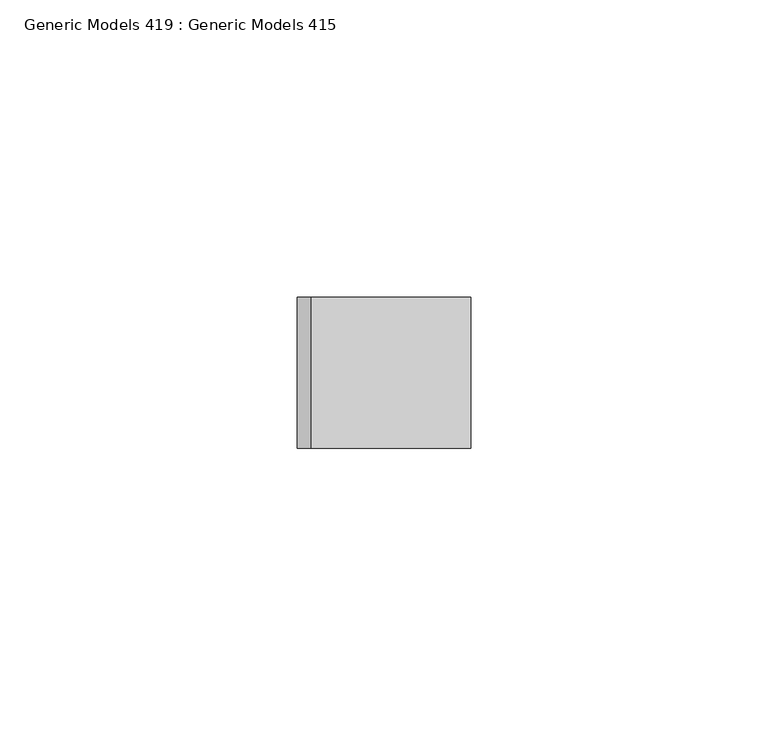
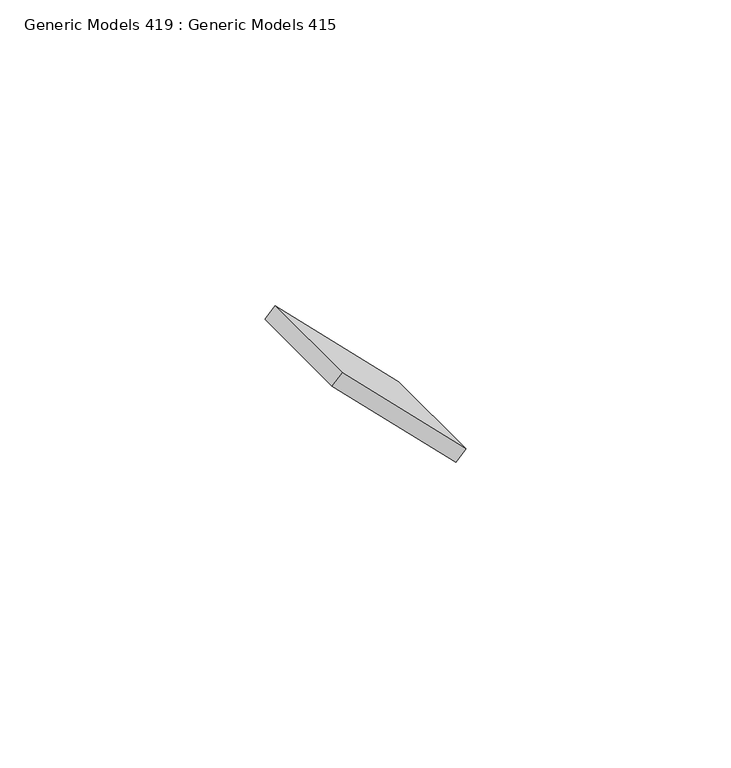
"""IFC4 building model written with IfcOpenShell, lengths in millimetres: proxy geometry, Generic Models 419 : Generic Models 415."""

from ifc_helpers import new_model, si_unit, frame, origin, place, context, project, spatial, polyline, outline, extrude, source, transform, mapped, element, save


def generic_models_419_generic_models_415_68036def(model_context):
    return source(origin(), model_context, "Body", "SweptSolid", [
        extrude(outline(polyline([(0.0, -38.1), (0.0, 0.0), (25.4, 0.0), (25.4, -38.1), (0.0, -38.1)])), frame((-6869.8996186, -4475.9863946, 128670.5002957), z_axis=(0.7071067811864907, 0.0, 0.7071067811866044), x_axis=(0.0, -1.0, 0.0)), (0.0, 0.0, 1.0), 3.175),
    ])


if __name__ == "__main__":
    model = new_model("IFC4")
    model_context = context("Model", 3, world=origin())
    ifc_project = project(units=[si_unit("LENGTHUNIT", "METRE", prefix="MILLI")], contexts=[model_context])
    site = spatial("IfcSite", under=ifc_project)
    building = spatial("IfcBuilding", under=site)
    placement = place(None, origin())
    generic_models_419_generic_models_415_shape = generic_models_419_generic_models_415_68036def(model_context)
    element("IfcBuildingElementProxy", 1, Name="Generic Models 419 : Generic Models 415", ObjectType="Generic Models 419 : Generic Models 415", at=placement, inside=building, context=model_context, shape_type="MappedRepresentation", body=[
        mapped(generic_models_419_generic_models_415_shape, transform((0.0, 0.0, 0.0), x_axis=(1.0, 0.0, 0.0), y_axis=(0.0, 1.0, 0.0), z_axis=(0.0, 0.0, 1.0))),
    ])
    save(model, "model.ifc")

# Revit data of these elements
# Element 1 (IfcBuildingElementProxy, "Generic Models 419 : Generic Models 415")
#   Materials on its faces: "_WELDED STEEL TABS FOR LOUVER ATTACHMENT"
# Materials
#   "_WELDED STEEL TABS FOR LOUVER ATTACHMENT": class "Metal", colour RGB 199 199 199, transparency 0, Description = "Structural steel 50ksi", Cost = 0
